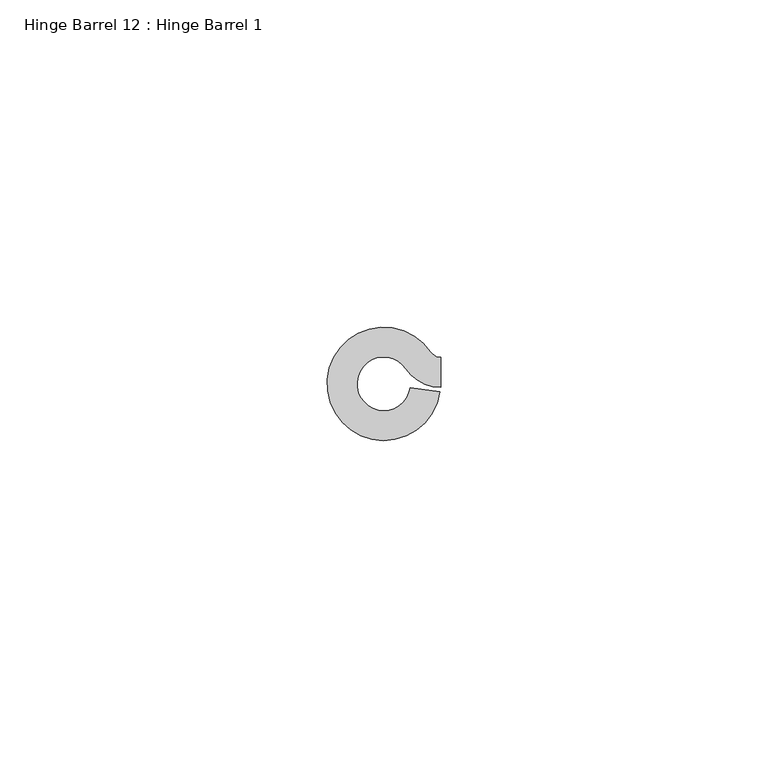
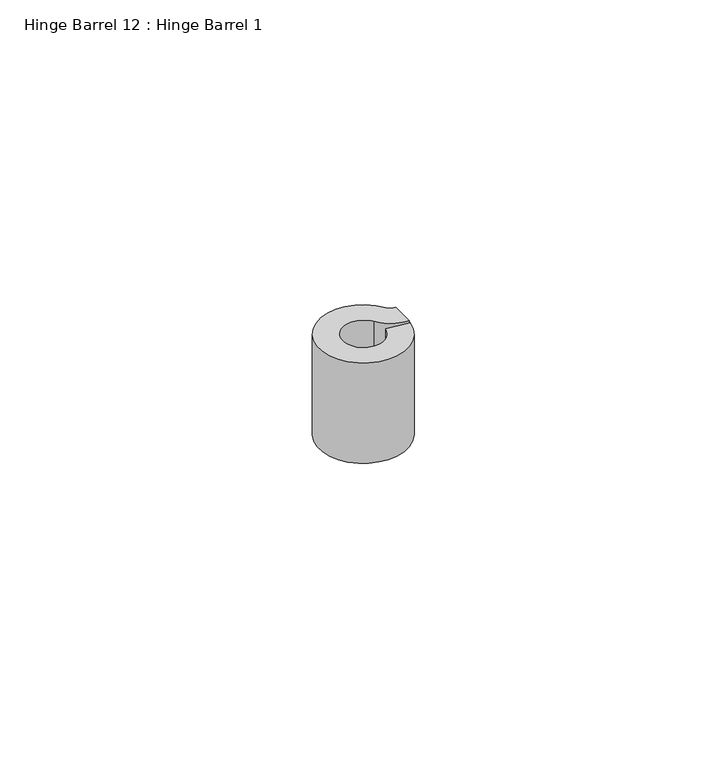
"""IFC4 building model written with IfcOpenShell, lengths in millimetres: proxy geometry, Hinge Barrel 12 : Hinge Barrel 1."""

from ifc_helpers import new_model, si_unit, point, frame, frame_2d, origin, place, context, project, spatial, polyline, circle_curve, trimmed, segment, composite_curve, outline, extrude, source, transform, mapped, element, save


def hinge_barrel_12_hinge_barrel_1_babfa127(model_context):
    return source(origin(), model_context, "Body", "SweptSolid", [
        extrude(outline(composite_curve([segment(trimmed(circle_curve(frame_2d((587319.1320739, -531776.6049841)), 4.0894), [point((587322.5194669, -531774.3139665))], [point((587323.1821338, -531777.1708529))], True, "CARTESIAN"), True, "CONTINUOUS"), segment(polyline([(587323.1821338, -531777.1708529), (587327.7022899, -531777.8024028)]), True, "CONTINUOUS"), segment(trimmed(circle_curve(frame_2d((587319.1320739, -531776.6049841)), 8.6534625), [point((587327.7022899, -531777.8024028))], [point((587326.3000393, -531771.7570273))], False, "CARTESIAN"), True, "CONTINUOUS"), segment(trimmed(circle_curve(frame_2d((587327.8245257, -531770.7259615)), 1.8404226), [point((587326.3000393, -531771.7570273))], [point((587327.8245257, -531772.5663841))], True, "CARTESIAN"), True, "CONTINUOUS"), segment(polyline([(587327.8245257, -531772.5663841), (587327.8245257, -531777.1304466)]), True, "CONTINUOUS"), segment(trimmed(circle_curve(frame_2d((587327.8245257, -531770.7259615)), 6.4044851), [point((587327.8245257, -531777.1304466))], [point((587322.5194669, -531774.3139665))], False, "CARTESIAN"), True, "CONTINUOUS")], self_intersect=False)), frame((0.0, 0.0, 2063.75), z_axis=(0.0, 0.0, 1.0), x_axis=(1.0, 0.0, 0.0)), (0.0, 0.0, 1.0), 20.8359375),
    ])


if __name__ == "__main__":
    model = new_model("IFC4")
    model_context = context("Model", 3, world=origin())
    ifc_project = project(units=[si_unit("LENGTHUNIT", "METRE", prefix="MILLI")], contexts=[model_context])
    site = spatial("IfcSite", under=ifc_project)
    building = spatial("IfcBuilding", under=site)
    placement = place(None, origin())
    hinge_barrel_12_hinge_barrel_1_shape = hinge_barrel_12_hinge_barrel_1_babfa127(model_context)
    element("IfcBuildingElementProxy", 1, Name="Hinge Barrel 12 : Hinge Barrel 1", ObjectType="Hinge Barrel 12 : Hinge Barrel 1", at=placement, inside=building, context=model_context, shape_type="MappedRepresentation", body=[
        mapped(hinge_barrel_12_hinge_barrel_1_shape, transform((0.0, 0.0, 0.0), x_axis=(1.0, 0.0, 0.0), y_axis=(0.0, 1.0, 0.0), z_axis=(0.0, 0.0, 1.0))),
    ])
    save(model, "model.ifc")

# Revit data of these elements
# Element 1 (IfcBuildingElementProxy, "Hinge Barrel 12 : Hinge Barrel 1")
#   Materials on its faces: "6\"X6\" WELD-ON STL BUTT HINGE"
# Materials
#   "6\"X6\" WELD-ON STL BUTT HINGE": class "Metal", colour RGB 189 187 185, transparency 0, Description = "Carbon steel", Cost = 0
